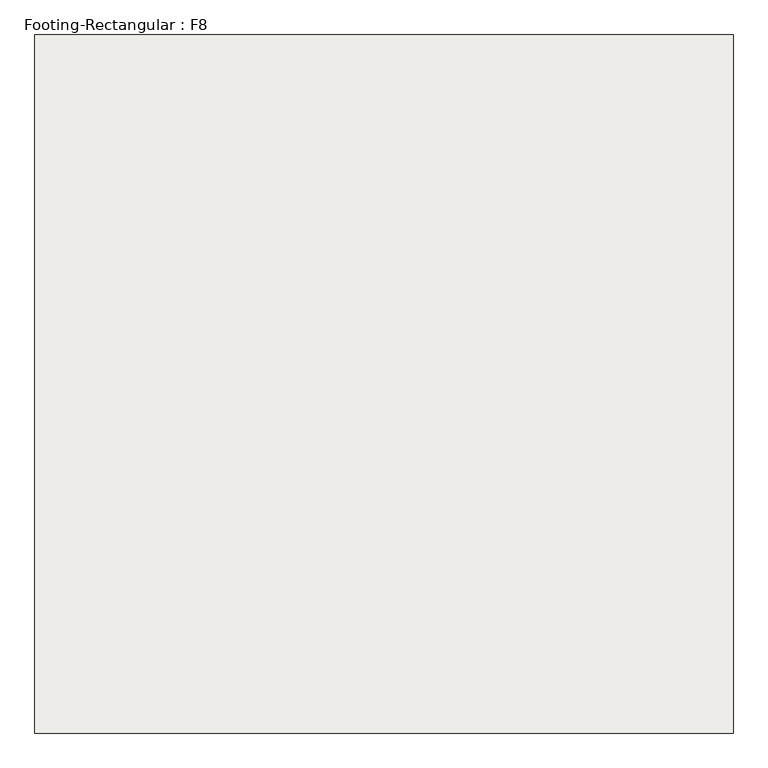
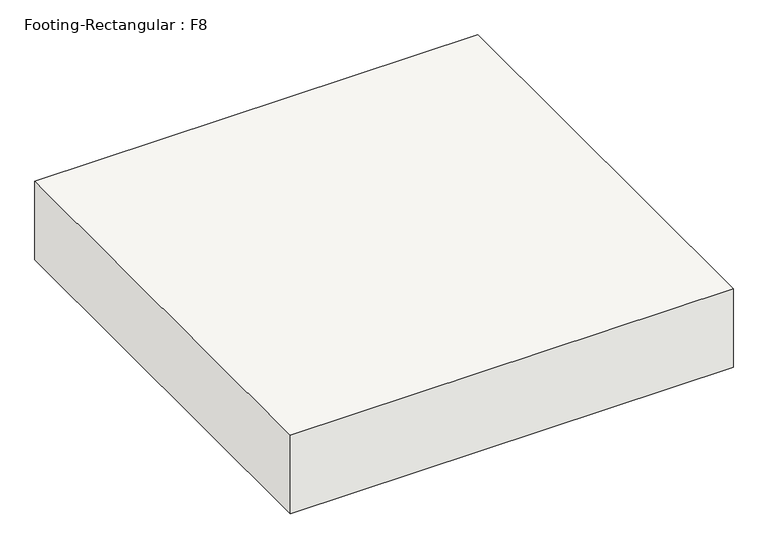
"""IFC4 building model written with IfcOpenShell, lengths in millimetres: slab geometry, Footing-Rectangular : F8."""

from ifc_helpers import new_model, si_unit, frame, origin, place, context, project, spatial, polyline, outline, extrude, source, transform, mapped, element, save


def footing_rectangular_f8_5614225c(model_context):
    return source(origin(), model_context, "Body", "SweptSolid", [
        extrude(outline(polyline([(1219.2, 1219.2), (1219.2, -1219.2), (-1219.2, -1219.2), (-1219.2, 1219.2), (1219.2, 1219.2)])), frame((0.0, 0.0, -457.2), z_axis=(0.0, 0.0, 1.0), x_axis=(1.0, 0.0, 0.0)), (0.0, 0.0, 1.0), 457.2),
    ])


if __name__ == "__main__":
    model = new_model("IFC4")
    model_context = context("Model", 3, world=origin())
    ifc_project = project(units=[si_unit("LENGTHUNIT", "METRE", prefix="MILLI")], contexts=[model_context])
    site = spatial("IfcSite", under=ifc_project)
    building = spatial("IfcBuilding", under=site)
    placement = place(None, origin())
    footing_rectangular_f8_shape = footing_rectangular_f8_5614225c(model_context)
    element("IfcSlab", 1, ObjectType="Footing-Rectangular : F8", at=placement, inside=building, context=model_context, shape_type="MappedRepresentation", body=[
        mapped(footing_rectangular_f8_shape, transform((0.0, 0.0, 0.0), x_axis=(1.0, 0.0, 0.0), y_axis=(0.0, 1.0, 0.0), z_axis=(0.0, 0.0, 1.0))),
    ])
    save(model, "model.ifc")

# Revit data of these elements
# Type "Footing-Rectangular : F8"
#   Assembly Code = "A1010100"
#   Width = 8' - 0"
#   Length = 8' - 0"
#   Foundation Thickness = 1' - 6"
#   Structural Material [instance default] = Concrete, Cast-in-Place gray
# Element 1 (IfcSlab, "Footing-Rectangular : F8")
#   Materials on its faces: "Concrete, Cast-in-Place gray"
# Materials
#   "Concrete, Cast-in-Place gray": class "Concrete", colour RGB 192 192 192, transparency 0, Description = "Cast-in-place concrete", Cost = 0
